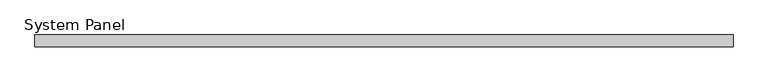
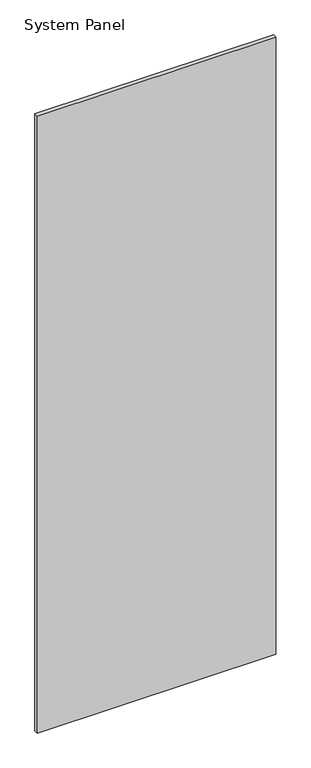
"""IFC4 building model written with IfcOpenShell, lengths in millimetres: plate geometry, System Panel : WWm-Glass-20mm-10mmOffset."""

from ifc_helpers import new_model, si_unit, origin, origin_with_axes, place, context, project, spatial, polyline, outline, extrude, source, transform, mapped, element, save


def system_panel_82a2c992(model_context):
    return source(origin(), model_context, "Body", "SweptSolid", [
        extrude(outline(polyline([(594.6105913, 0.0), (-594.6105913, 0.0), (-594.6105913, 20.0), (594.6105913, 20.0), (594.6105913, 0.0)])), origin_with_axes(), (0.0, 0.0, 1.0), 3250.0),
    ])


if __name__ == "__main__":
    model = new_model("IFC4")
    model_context = context("Model", 3, world=origin())
    ifc_project = project(units=[si_unit("LENGTHUNIT", "METRE", prefix="MILLI")], contexts=[model_context])
    site = spatial("IfcSite", under=ifc_project)
    building = spatial("IfcBuilding", under=site)
    placement = place(None, origin())
    system_panel_shape = system_panel_82a2c992(model_context)
    element("IfcPlate", 1, ObjectType="System Panel : WWm-Glass-20mm-10mmOffset", at=placement, inside=building, context=model_context, shape_type="MappedRepresentation", body=[
        mapped(system_panel_shape, transform((0.0, 0.0, 0.0), x_axis=(1.0, 0.0, 0.0), y_axis=(0.0, 1.0, 0.0), z_axis=(0.0, 0.0, 1.0))),
    ])
    save(model, "model.ifc")

# Revit data of these elements
# Type "System Panel : WWm-Glass-20mm-10mmOffset"
#   Finish = ""
# Element 1 (IfcPlate, "System Panel : WWm-Glass-20mm-10mmOffset")
#   Materials on its faces: "WW-EC-GL-Storefront"
# Materials
#   "WW-EC-GL-Storefront": class "Glass", colour RGB 236 240 239, transparency 0.85, Description = "Storefront Glass", Cost = 0
